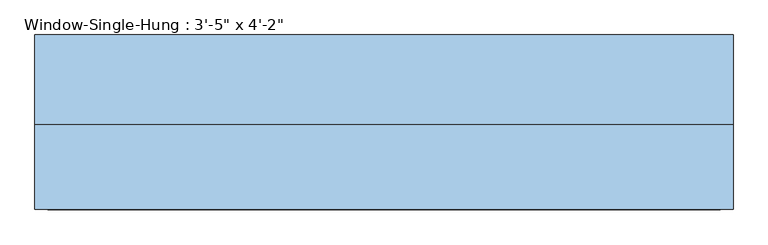
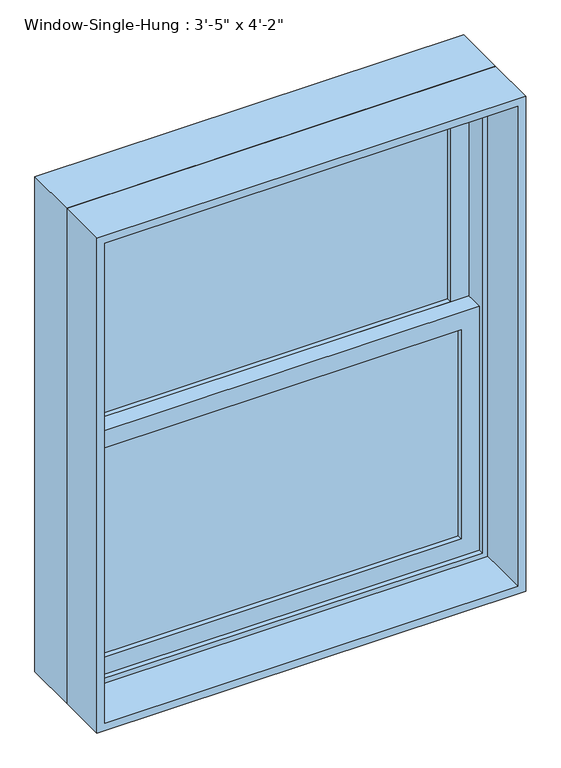
"""IFC4 building model written with IfcOpenShell, lengths in millimetres: window geometry."""

from ifc_helpers import new_model, si_unit, frame, origin, place, context, project, spatial, polyline, outline, extrude, source, transform, mapped, element, save


def window_7112179c(model_context):
    return source(origin(), model_context, "Body", "SweptSolid", [
        extrude(outline(polyline([(444.5, 50.8), (444.5, 44.45), (-444.5, 44.45), (-444.5, 50.8), (444.5, 50.8)])), frame((0.0, 0.0, 990.6), z_axis=(0.0, 0.0, 1.0), x_axis=(1.0, 0.0, 0.0)), (0.0, 0.0, 1.0), 536.575),
        extrude(outline(polyline([(-444.5, 38.1), (444.5, 38.1), (444.5, 31.75), (-444.5, 31.75), (-444.5, 38.1)])), frame((0.0, 0.0, 990.6), z_axis=(0.0, 0.0, 1.0), x_axis=(1.0, 0.0, 0.0)), (0.0, 0.0, 1.0), 536.575),
        extrude(outline(polyline([(444.5, 95.25), (444.5, 88.9), (-444.5, 88.9), (-444.5, 95.25), (444.5, 95.25)])), frame((0.0, 0.0, 1571.625), z_axis=(0.0, 0.0, 1.0), x_axis=(1.0, 0.0, 0.0)), (0.0, 0.0, 1.0), 536.575),
        extrude(outline(polyline([(-444.5, 82.55), (444.5, 82.55), (444.5, 76.2), (-444.5, 76.2), (-444.5, 82.55)])), frame((0.0, 0.0, 1571.625), z_axis=(0.0, 0.0, 1.0), x_axis=(1.0, 0.0, 0.0)), (0.0, 0.0, 1.0), 536.575),
        extrude(outline(polyline([(1571.625, -488.95), (946.15, -488.95), (946.15, 488.95), (1571.625, 488.95), (1571.625, -488.95)]), holes=[polyline([(1527.175, 444.5), (990.6, 444.5), (990.6, -444.5), (1527.175, -444.5), (1527.175, 444.5)])]), frame((0.0, 19.05, 0.0), z_axis=(0.0, 1.0, 0.0), x_axis=(0.0, 0.0, 1.0)), (0.0, 0.0, 1.0), 44.45),
        extrude(outline(polyline([(2152.65, -488.95), (1527.175, -488.95), (1527.175, 488.95), (2152.65, 488.95), (2152.65, -488.95)]), holes=[polyline([(2108.2, 444.5), (1571.625, 444.5), (1571.625, -444.5), (2108.2, -444.5), (2108.2, 444.5)])]), frame((0.0, 63.5, 0.0), z_axis=(0.0, 1.0, 0.0), x_axis=(0.0, 0.0, 1.0)), (0.0, 0.0, 1.0), 44.45),
        extrude(outline(polyline([(2184.4, -520.7), (914.4, -520.7), (914.4, 520.7), (2184.4, 520.7), (2184.4, -520.7)]), holes=[polyline([(2152.65, 488.95), (946.15, 488.95), (946.15, -488.95), (2152.65, -488.95), (2152.65, 488.95)])]), frame((0.0, 6.35, 0.0), z_axis=(0.0, 1.0, 0.0), x_axis=(0.0, 0.0, 1.0)), (0.0, 0.0, 1.0), 133.35),
        extrude(outline(polyline([(2184.4, 520.7), (2184.4, -520.7), (914.4, -520.7), (914.4, 520.7), (2184.4, 520.7)]), holes=[polyline([(2165.35, 501.65), (933.45, 501.65), (933.45, -501.65), (2165.35, -501.65), (2165.35, 501.65)])]), frame((0.0, -120.65, 0.0), z_axis=(0.0, 1.0, 0.0), x_axis=(0.0, 0.0, 1.0)), (0.0, 0.0, 1.0), 127.0),
    ])


if __name__ == "__main__":
    model = new_model("IFC4")
    model_context = context("Model", 3, world=origin())
    ifc_project = project(units=[si_unit("LENGTHUNIT", "METRE", prefix="MILLI")], contexts=[model_context])
    site = spatial("IfcSite", under=ifc_project)
    building = spatial("IfcBuilding", under=site)
    placement = place(None, origin())
    window_shape = window_7112179c(model_context)
    element("IfcWindow", 1, ObjectType="Window-Single-Hung : 3'-5\" x 4'-2\"", at=placement, inside=building, context=model_context, shape_type="MappedRepresentation", body=[
        mapped(window_shape, transform((0.0, 0.0, 0.0), x_axis=(1.0, 0.0, 0.0), y_axis=(0.0, 1.0, 0.0), z_axis=(0.0, 0.0, 1.0))),
    ])
    save(model, "model.ifc")

# Revit data of these elements
# Type "Window-Single-Hung : 3'-5\" x 4'-2\""
#   Type Mark = "06"
#   Fire Rating = "0.5h"
#   Construction Type Id = "DG-DR"
#   Assembly Code = "B2020100"
#   Analytic Construction = "Double glazing - domestic"
#   Wall Thickness [instance default] = 0' - 6"
#   Window Inset [instance default] = 0' - 0"
#   Visual Light Transmittance = 0.81
#   Thermal Resistance (R) = 0.319569 (m²·K)/W
#   Solar Heat Gain Coefficient = 0.76
#   Muntin Width = 2' - 11"
#   Muntin Height = 1' - 9 1/8"
#   Interior Wall Closure [instance default] = 0' - 1 1/2"
#   Rough Width = 3' - 5 1/2"
#   Rough Height = 4' - 2 1/2"
#   Frame Extension [instance default] = 0' - 1 1/4"
#   Exterior Wall Closure [instance default] = 0' - 0 1/2"
#   Extension Jamb [instance default] = 0' - 1 1/2"
#   Heat Transfer Coefficient (U) = 3.12929 W/(m²·K)
#   Height = 4' - 2"
#   Width = 3' - 5"
#   Top Muntin Visibility = no
#   Indicator Visibility = no
#   Extension Jamb Visibility [instance default] = yes
#   Interior Trim Visibility [instance default] = yes
#   Exterior Trim Visibility [instance default] = yes
#   Bottom Muntin Visibility = no
#   Muntin Pattern = Muntin Pattern_2x2 : Muntin Pattern_2x2
#   Interior Trim Material = 1X WOOD COMPOSITE TRIM
#   Interior Trim = Trim-Window-Interior-Flat : Picture Frame
#   Exterior Trim Material = 1X WOOD COMPOSITE TRIM
#   Exterior Trim = Trim-Window-Exterior-Flat : with Sill
#   Glass Panel Material = NEW DOUBLE HUNG WINDOWS (TYP.)
#   Exterior Frame Material = 1X WOOD COMPOSITE TRIM
#   Interior Frame Material = 1X WOOD COMPOSITE TRIM
#   Wall Closure = (empty or 0)
# Element 1 (IfcWindow, "Window-Single-Hung : 3'-5\" x 4'-2\"")
#   Wall Thickness = 0' - 9 1/2"
#   Extension Jamb = 0' - 5"
#   Materials on its faces: "1X WOOD COMPOSITE TRIM", "NEW DOUBLE HUNG WINDOWS (TYP.)"
# Materials
#   "1X WOOD COMPOSITE TRIM": class "Generic", colour RGB 88 61 61, transparency 0, Cost = 0
#   "NEW DOUBLE HUNG WINDOWS (TYP.)": class "Glass", colour RGB 218 227 224, transparency 0.85, Description = "Soda Lime Glass", Cost = 0
